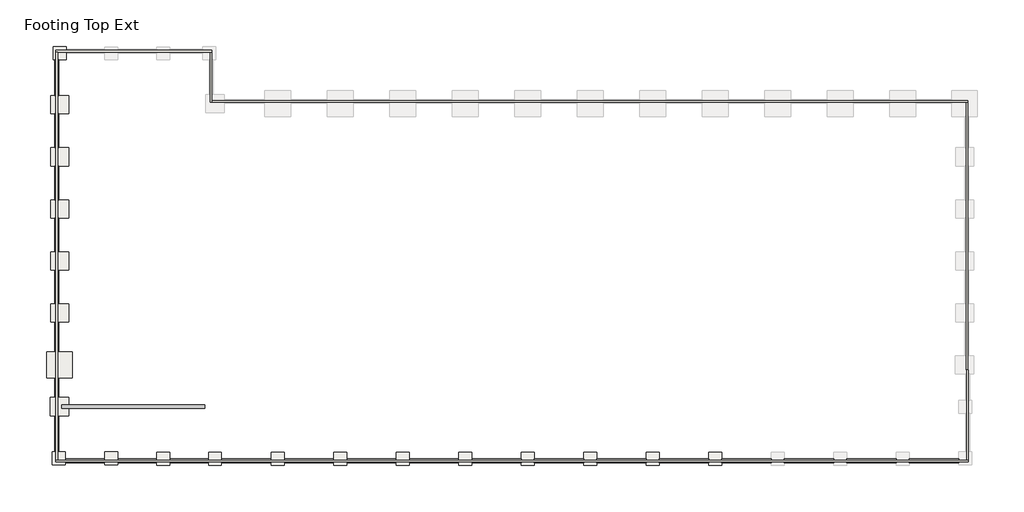
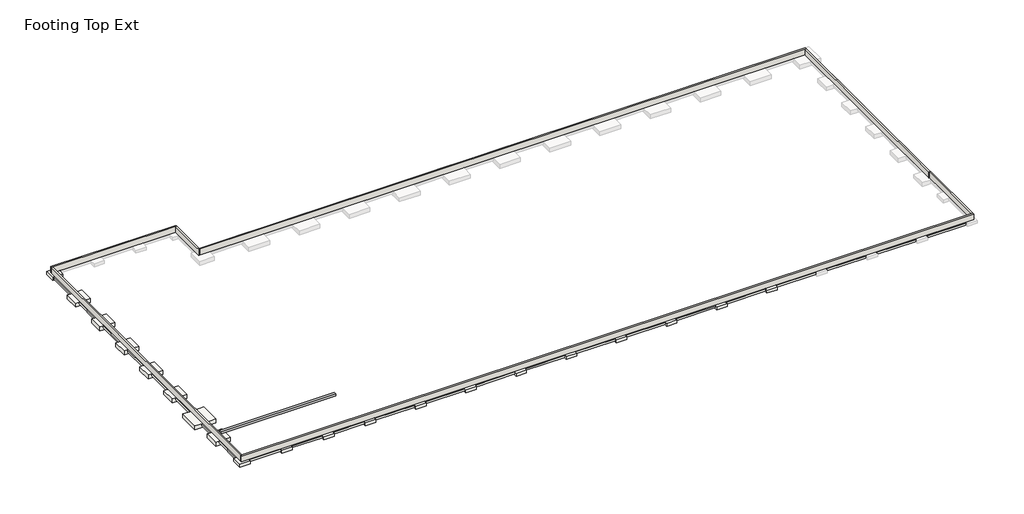
# One storey, part 1 of 2: 20 slabs, 7 walls, 2 footings, 1 beam.
"""IFC4 building model written with IfcOpenShell, lengths in millimetres."""

import ifcopenshell
import ifcopenshell.guid

model = None  # the IFC model being written
_history = None  # IfcOwnerHistory: only IFC2X3 demands one
_inside = {}  # id of a spatial element -> (the spatial element, [elements in it])
_under = {}  # id of a project, library or spatial element -> (it, [spatial elements below it])
_declared = {}  # id of a project -> (the project, [libraries it declares])
_typed = {}  # id of a type object -> (the type object, [elements of that type])
_made_of = {}  # id of a material, layer set ... -> (it, [elements and type objects made of it])


def new_model(schema):
    """Start an empty IFC model of exactly this schema.

    Asked for "IFC4X3", IfcOpenShell would pick the latest addendum, in which some entities
    have other attributes; the version numbers below select the first issue.
    IFC2X3 requires an IfcOwnerHistory on every rooted entity: one is made here for all.
    """
    global model, _history
    if schema == "IFC4X3":
        model = ifcopenshell.file(schema_version=(4, 3, 0, 0))
    else:
        model = ifcopenshell.file(schema=schema)
    _inside.clear()
    _under.clear()
    _declared.clear()
    _typed.clear()
    _made_of.clear()
    _history = None
    if model.schema == "IFC2X3":
        org = make("IfcOrganization", Name="unknown")
        user = make(
            "IfcPersonAndOrganization",
            ThePerson=make("IfcPerson", FamilyName="unknown"),
            TheOrganization=org,
        )
        app = make(
            "IfcApplication",
            ApplicationDeveloper=org,
            Version="unknown",
            ApplicationFullName="unknown",
            ApplicationIdentifier="unknown",
        )
        _history = make(
            "IfcOwnerHistory",
            OwningUser=user,
            OwningApplication=app,
            ChangeAction="ADDED",
            CreationDate=0,
        )
    return model


def make(cls, **values):
    """One entity of the class cls with the attributes given. An attribute that is None is left unset."""
    return model.create_entity(
        cls, **{name: value for name, value in values.items() if value is not None}
    )


def rooted(cls, **values):
    """An entity with a GlobalId (a new one), such as an element, a storey or a relation."""
    return make(cls, GlobalId=ifcopenshell.guid.new(), OwnerHistory=_history, **values)


def si_unit(unit_type, name, prefix=None):
    """IfcSIUnit, for example si_unit("LENGTHUNIT", "METRE", prefix="MILLI")."""
    return make("IfcSIUnit", UnitType=unit_type, Prefix=prefix, Name=name)


def assignment(units):
    """IfcUnitAssignment: the units of a project."""
    return None if units is None else make("IfcUnitAssignment", Units=units)


def point(xyz):
    """IfcCartesianPoint."""
    return None if xyz is None else make("IfcCartesianPoint", Coordinates=xyz)


def direction(xyz):
    """IfcDirection."""
    return None if xyz is None else make("IfcDirection", DirectionRatios=xyz)


def frame(location, z_axis=None, x_axis=None):
    """IfcAxis2Placement3D, a coordinate frame: its origin and axes. An axis left out is left unset."""
    return make(
        "IfcAxis2Placement3D",
        Location=point(location),
        Axis=direction(z_axis),
        RefDirection=direction(x_axis),
    )


def origin():
    """The frame at (0, 0, 0) with its axes left unset."""
    return frame((0.0, 0.0, 0.0))


def place(relative_to, where):
    """IfcLocalPlacement: puts the frame where relative to a parent placement (None: the world)."""
    return make(
        "IfcLocalPlacement", PlacementRelTo=relative_to, RelativePlacement=where
    )


def context(
    kind, dimensions, precision=None, world=None, true_north=None, identifier=None
):
    """IfcGeometricRepresentationContext, for example the 3D "Model" context."""
    return make(
        "IfcGeometricRepresentationContext",
        ContextIdentifier=identifier,
        ContextType=kind,
        CoordinateSpaceDimension=dimensions,
        Precision=precision,
        WorldCoordinateSystem=world,
        TrueNorth=true_north,
    )


def project(units=None, contexts=None):
    """IfcProject with its units and contexts."""
    return rooted(
        "IfcProject",
        Name="project",
        RepresentationContexts=contexts,
        UnitsInContext=assignment(units),
    )


def spatial(cls, under=None, at=None, **own):
    """A site, building, storey or space (cls), placed at a placement, below another one or the project."""
    s = rooted(cls, ObjectPlacement=at, **own)
    if under is not None:
        _under.setdefault(under.id(), (under, []))[1].append(s)
    return s


def polyline(points):
    """IfcPolyline through the points."""
    return make("IfcPolyline", Points=[point(p) for p in points])


def outline(outer, holes=None, kind="AREA"):
    """IfcArbitraryClosedProfileDef: a profile drawn as a closed curve; with holes, ...WithVoids."""
    if holes is None:
        return make("IfcArbitraryClosedProfileDef", ProfileType=kind, OuterCurve=outer)
    return make(
        "IfcArbitraryProfileDefWithVoids",
        ProfileType=kind,
        OuterCurve=outer,
        InnerCurves=holes,
    )


def extrude(swept, where, along, depth):
    """IfcExtrudedAreaSolid: the profile swept, set in the frame where, extruded along a direction by depth."""
    return make(
        "IfcExtrudedAreaSolid",
        SweptArea=swept,
        Position=where,
        ExtrudedDirection=direction(along),
        Depth=depth,
    )


def faces_of(points, faces, orient=None, outer=None):
    """IfcFace entities. A face is a list of loops; a loop is a list of indices into points, from 0.

    orient and outer hold one flag for each loop. By default every Orientation is true, the
    first loop of a face is its IfcFaceOuterBound and the others are IfcFaceBound.
    """
    made = []
    for i, loops in enumerate(faces):
        bounds = []
        for j, loop in enumerate(loops):
            is_outer = j == 0 if outer is None else outer[i][j]
            bounds.append(
                make(
                    "IfcFaceOuterBound" if is_outer else "IfcFaceBound",
                    Bound=make("IfcPolyLoop", Polygon=[points[k] for k in loop]),
                    Orientation=True if orient is None else orient[i][j],
                )
            )
        made.append(make("IfcFace", Bounds=bounds))
    return made


def faceted_brep(points, faces, orient=None, outer=None, voids=None):
    """IfcFacetedBrep: a solid bounded by flat faces; with voids (closed shells), ...WithVoids."""
    shared = [point(p) for p in points]
    hull = make("IfcClosedShell", CfsFaces=faces_of(shared, faces, orient, outer))
    if voids is None:
        return make("IfcFacetedBrep", Outer=hull)
    return make(
        "IfcFacetedBrepWithVoids",
        Outer=hull,
        Voids=[
            make(cls, CfsFaces=faces_of(shared, fs, o, b)) for cls, fs, o, b in voids
        ],
    )


def shape(context_of_items, identifier, shape_type, items):
    """IfcShapeRepresentation: the items that make up one representation, for example the "Body"."""
    return make(
        "IfcShapeRepresentation",
        ContextOfItems=context_of_items,
        RepresentationIdentifier=identifier,
        RepresentationType=shape_type,
        Items=items,
    )


def made_of(thing, what):
    """Note that an element or type object is made of a material, layer set ...; save() writes the relation."""
    if what is not None:
        _made_of.setdefault(what.id(), (what, []))[1].append(thing)
    return thing


def element(
    cls,
    number,
    at=None,
    inside=None,
    cuts=None,
    type_object=None,
    material=None,
    context=None,
    identifier="Body",
    shape_type=None,
    held_by="IfcProductDefinitionShape",
    body=None,
    shapes=None,
    **own,
):
    """One element of the class cls, such as IfcWall. Its Tag is "e" and its number.

    at: its placement. inside: the storey or other place that contains it. cuts: it is an
    opening in that element (IfcRelVoidsElement). A single representation is given by context,
    identifier, shape_type and body (its items); several are given by shapes. held_by: the class
    of the entity that holds the representations. save() writes the other relations.
    """
    e = rooted(cls, Tag="e%d" % number, ObjectPlacement=at, **own)
    if body is not None:
        shapes = [shape(context, identifier, shape_type, body)]
    if shapes is not None:
        e.Representation = make(held_by, Representations=shapes)
    if inside is not None:
        _inside.setdefault(inside.id(), (inside, []))[1].append(e)
    if cuts is not None:
        rooted(
            "IfcRelVoidsElement", RelatingBuildingElement=cuts, RelatedOpeningElement=e
        )
    if type_object is not None:
        _typed.setdefault(type_object.id(), (type_object, []))[1].append(e)
    return made_of(e, material)


def aggregate(whole, parts):
    """IfcRelAggregates: a whole, such as a stair, and the parts it consists of."""
    return rooted("IfcRelAggregates", RelatingObject=whole, RelatedObjects=parts)


def save(model, path):
    """Write the relations noted so far, then the file.

    IfcRelAggregates (storeys below a building ...), IfcRelContainedInSpatialStructure (elements
    in a storey), IfcRelDefinesByType, IfcRelAssociatesMaterial and IfcRelDeclares: one each for
    every whole, place, type object, material and project.
    """
    for whole, parts in _under.values():
        aggregate(whole, parts)
    for where, things in _inside.values():
        rooted(
            "IfcRelContainedInSpatialStructure",
            RelatedElements=things,
            RelatingStructure=where,
        )
    for kind, things in _typed.values():
        rooted("IfcRelDefinesByType", RelatedObjects=things, RelatingType=kind)
    for what, things in _made_of.values():
        rooted("IfcRelAssociatesMaterial", RelatedObjects=things, RelatingMaterial=what)
    for by, libraries in _declared.values():
        rooted("IfcRelDeclares", RelatingContext=by, RelatedDefinitions=libraries)
    model.write(path)


model = new_model("IFC4")

# Units and contexts
model_context = context("Model", 3, world=origin())
ifc_project = project(units=[si_unit("LENGTHUNIT", "METRE", prefix="MILLI")], contexts=[model_context])

# Site, building, storey
site = spatial("IfcSite", under=ifc_project)
building = spatial("IfcBuilding", under=site)
storey = spatial("IfcBuildingStorey", under=building, Name="Footing Top Ext", Elevation=-914.4)

# Beam
placement = place(None, origin())
element("IfcBeam", 1, ObjectType="Concrete-Rectangular Beam : 16 x 12", at=placement, inside=storey, context=model_context, shape_type="SweptSolid", body=[
    extrude(outline(polyline([(321987.9648264, -572404.4391729), (321987.9648264, -572810.8391729), (305208.0898264, -572810.8391729), (305208.0898264, -572404.4391729), (321987.9648264, -572404.4391729)])), frame((0.0, 0.0, -609.6), z_axis=(0.0, 0.0, 1.0), x_axis=(1.0, 0.0, 0.0)), (0.0, 0.0, 1.0), 304.8),
])

# Footings
element("IfcFooting", 2, ObjectType="Bearing Footing - 18\" x 12\"", at=placement, inside=storey, context=model_context, shape_type="SweptSolid", body=[
    extrude(outline(polyline([(305608.1398264, -579216.5913841), (305608.1398264, -578759.3913841), (310230.9398264, -578759.3913841), (310230.9398264, -579216.5913841), (305608.1398264, -579216.5913841)])), frame((0.0, 0.0, -1219.2), z_axis=(0.0, 0.0, 1.0), x_axis=(1.0, 0.0, 0.0)), (0.0, 0.0, 1.0), 304.8),
    extrude(outline(polyline([(311754.9398264, -579216.5913841), (311754.9398264, -578759.3913841), (316361.8648264, -578759.3913841), (316361.8648264, -579216.5913841), (311754.9398264, -579216.5913841)])), frame((0.0, 0.0, -1219.2), z_axis=(0.0, 0.0, 1.0), x_axis=(1.0, 0.0, 0.0)), (0.0, 0.0, 1.0), 304.8),
    extrude(outline(polyline([(317885.8648264, -579216.5913841), (317885.8648264, -578759.3913841), (322457.8648264, -578759.3913841), (322457.8648264, -579216.5913841), (317885.8648264, -579216.5913841)])), frame((0.0, 0.0, -1219.2), z_axis=(0.0, 0.0, 1.0), x_axis=(1.0, 0.0, 0.0)), (0.0, 0.0, 1.0), 304.8),
    extrude(outline(polyline([(323981.8648264, -579216.5913841), (323981.8648264, -578759.3913841), (329839.7398264, -578759.3913841), (329839.7398264, -579216.5913841), (323981.8648264, -579216.5913841)])), frame((0.0, 0.0, -1219.2), z_axis=(0.0, 0.0, 1.0), x_axis=(1.0, 0.0, 0.0)), (0.0, 0.0, 1.0), 304.8),
    extrude(outline(polyline([(331363.7398264, -579216.5913841), (331363.7398264, -578759.3913841), (337193.0398264, -578759.3913841), (337193.0398264, -579216.5913841), (331363.7398264, -579216.5913841)])), frame((0.0, 0.0, -1219.2), z_axis=(0.0, 0.0, 1.0), x_axis=(1.0, 0.0, 0.0)), (0.0, 0.0, 1.0), 304.8),
    extrude(outline(polyline([(338717.0398264, -579216.5913841), (338717.0398264, -578759.3913841), (344546.3398264, -578759.3913841), (344546.3398264, -579216.5913841), (338717.0398264, -579216.5913841)])), frame((0.0, 0.0, -1219.2), z_axis=(0.0, 0.0, 1.0), x_axis=(1.0, 0.0, 0.0)), (0.0, 0.0, 1.0), 304.8),
    extrude(outline(polyline([(346070.3398264, -579216.5913841), (346070.3398264, -578759.3913841), (351899.6398264, -578759.3913841), (351899.6398264, -579216.5913841), (346070.3398264, -579216.5913841)])), frame((0.0, 0.0, -1219.2), z_axis=(0.0, 0.0, 1.0), x_axis=(1.0, 0.0, 0.0)), (0.0, 0.0, 1.0), 304.8),
    extrude(outline(polyline([(353423.6398264, -579216.5913841), (353423.6398264, -578759.3913841), (359252.9398264, -578759.3913841), (359252.9398264, -579216.5913841), (353423.6398264, -579216.5913841)])), frame((0.0, 0.0, -1219.2), z_axis=(0.0, 0.0, 1.0), x_axis=(1.0, 0.0, 0.0)), (0.0, 0.0, 1.0), 304.8),
    extrude(outline(polyline([(360776.9398264, -579216.5913841), (360776.9398264, -578759.3913841), (366606.2398264, -578759.3913841), (366606.2398264, -579216.5913841), (360776.9398264, -579216.5913841)])), frame((0.0, 0.0, -1219.2), z_axis=(0.0, 0.0, 1.0), x_axis=(1.0, 0.0, 0.0)), (0.0, 0.0, 1.0), 304.8),
    extrude(outline(polyline([(368130.2398264, -579216.5913841), (368130.2398264, -578759.3913841), (373959.5398264, -578759.3913841), (373959.5398264, -579216.5913841), (368130.2398264, -579216.5913841)])), frame((0.0, 0.0, -1219.2), z_axis=(0.0, 0.0, 1.0), x_axis=(1.0, 0.0, 0.0)), (0.0, 0.0, 1.0), 304.8),
    extrude(outline(polyline([(375483.5398264, -579216.5913841), (375483.5398264, -578759.3913841), (381312.8398264, -578759.3913841), (381312.8398264, -579216.5913841), (375483.5398264, -579216.5913841)])), frame((0.0, 0.0, -1219.2), z_axis=(0.0, 0.0, 1.0), x_axis=(1.0, 0.0, 0.0)), (0.0, 0.0, 1.0), 304.8),
    extrude(outline(polyline([(382836.8398264, -579216.5913841), (382836.8398264, -578759.3913841), (388666.1398264, -578759.3913841), (388666.1398264, -579216.5913841), (382836.8398264, -579216.5913841)])), frame((0.0, 0.0, -1219.2), z_axis=(0.0, 0.0, 1.0), x_axis=(1.0, 0.0, 0.0)), (0.0, 0.0, 1.0), 304.8),
    extrude(outline(polyline([(390190.1398264, -579216.5913841), (390190.1398264, -578759.3913841), (396019.4398264, -578759.3913841), (396019.4398264, -579216.5913841), (390190.1398264, -579216.5913841)])), frame((0.0, 0.0, -1219.2), z_axis=(0.0, 0.0, 1.0), x_axis=(1.0, 0.0, 0.0)), (0.0, 0.0, 1.0), 304.8),
    extrude(outline(polyline([(397543.4398264, -579216.5913841), (397543.4398264, -578759.3913841), (403372.7398264, -578759.3913841), (403372.7398264, -579216.5913841), (397543.4398264, -579216.5913841)])), frame((0.0, 0.0, -1219.2), z_axis=(0.0, 0.0, 1.0), x_axis=(1.0, 0.0, 0.0)), (0.0, 0.0, 1.0), 304.8),
    extrude(outline(polyline([(404896.7398264, -579216.5913841), (404896.7398264, -578759.3913841), (410700.6398264, -578759.3913841), (410700.6398264, -579216.5913841), (404896.7398264, -579216.5913841)])), frame((0.0, 0.0, -1219.2), z_axis=(0.0, 0.0, 1.0), x_axis=(1.0, 0.0, 0.0)), (0.0, 0.0, 1.0), 304.8),
])
element("IfcFooting", 3, ObjectType="Bearing Footing - 18\" x 12\"", at=placement, inside=storey, context=model_context, shape_type="SweptSolid", body=[
    extrude(outline(polyline([(304369.8898264, -531712.2413841), (304827.0898264, -531712.2413841), (304827.0898264, -535985.7913841), (304369.8898264, -535985.7913841), (304369.8898264, -531712.2413841)])), frame((0.0, 0.0, -1219.2), z_axis=(0.0, 0.0, 1.0), x_axis=(1.0, 0.0, 0.0)), (0.0, 0.0, 1.0), 304.8),
    extrude(outline(polyline([(304369.8898264, -538119.3913841), (304827.0898264, -538119.3913841), (304827.0898264, -542113.5413841), (304369.8898264, -542113.5413841), (304369.8898264, -538119.3913841)])), frame((0.0, 0.0, -1219.2), z_axis=(0.0, 0.0, 1.0), x_axis=(1.0, 0.0, 0.0)), (0.0, 0.0, 1.0), 304.8),
    extrude(outline(polyline([(304369.8898264, -544247.1413841), (304827.0898264, -544247.1413841), (304827.0898264, -548241.2913841), (304369.8898264, -548241.2913841), (304369.8898264, -544247.1413841)])), frame((0.0, 0.0, -1219.2), z_axis=(0.0, 0.0, 1.0), x_axis=(1.0, 0.0, 0.0)), (0.0, 0.0, 1.0), 304.8),
    extrude(outline(polyline([(304369.8898264, -550374.8913841), (304827.0898264, -550374.8913841), (304827.0898264, -554369.0413841), (304369.8898264, -554369.0413841), (304369.8898264, -550374.8913841)])), frame((0.0, 0.0, -1219.2), z_axis=(0.0, 0.0, 1.0), x_axis=(1.0, 0.0, 0.0)), (0.0, 0.0, 1.0), 304.8),
    extrude(outline(polyline([(304369.8898264, -556502.6413841), (304827.0898264, -556502.6413841), (304827.0898264, -560496.7913841), (304369.8898264, -560496.7913841), (304369.8898264, -556502.6413841)])), frame((0.0, 0.0, -1219.2), z_axis=(0.0, 0.0, 1.0), x_axis=(1.0, 0.0, 0.0)), (0.0, 0.0, 1.0), 304.8),
    extrude(outline(polyline([(304369.8898264, -562630.3913841), (304827.0898264, -562630.3913841), (304827.0898264, -566167.3413841), (304369.8898264, -566167.3413841), (304369.8898264, -562630.3913841)])), frame((0.0, 0.0, -1219.2), z_axis=(0.0, 0.0, 1.0), x_axis=(1.0, 0.0, 0.0)), (0.0, 0.0, 1.0), 304.8),
    extrude(outline(polyline([(304369.8898264, -569215.3413841), (304827.0898264, -569215.3413841), (304827.0898264, -571526.7413841), (304369.8898264, -571526.7413841), (304369.8898264, -569215.3413841)])), frame((0.0, 0.0, -1219.2), z_axis=(0.0, 0.0, 1.0), x_axis=(1.0, 0.0, 0.0)), (0.0, 0.0, 1.0), 304.8),
    extrude(outline(polyline([(304369.8898264, -573660.3413841), (304827.0898264, -573660.3413841), (304827.0898264, -577933.8913841), (304369.8898264, -577933.8913841), (304369.8898264, -573660.3413841)])), frame((0.0, 0.0, -1219.2), z_axis=(0.0, 0.0, 1.0), x_axis=(1.0, 0.0, 0.0)), (0.0, 0.0, 1.0), 304.8),
])

# Slabs
element("IfcSlab", 4, ObjectType="Footing-Rectangular : F10", at=placement, inside=storey, context=model_context, shape_type="Brep", body=[
    faceted_brep([(306452.6898264, -566167.3413841, -914.4), (304827.0898264, -566167.3413841, -914.4), (304369.8898264, -566167.3413841, -914.4), (303404.6898264, -566167.3413841, -914.4), (303404.6898264, -569215.3413841, -914.4), (304369.8898264, -569215.3413841, -914.4), (304827.0898264, -569215.3413841, -914.4), (306452.6898264, -569215.3413841, -914.4), (306452.6898264, -566167.3413841, -1524.0), (306452.6898264, -569215.3413841, -1524.0), (303404.6898264, -569215.3413841, -1524.0), (303404.6898264, -566167.3413841, -1524.0)], [[[0, 1, 2, 3, 4, 5, 6, 7]], [[8, 9, 10, 11]], [[3, 2, 1, 0, 8, 11]], [[4, 3, 11, 10]], [[7, 6, 5, 4, 10, 9]], [[0, 7, 9, 8]]]),
])
element("IfcSlab", 5, ObjectType="Footing-Rectangular : F5", at=placement, inside=storey, context=model_context, shape_type="Brep", body=[
    faceted_brep([(305697.0398264, -530188.2413841, -914.4), (304173.0398264, -530188.2413841, -914.4), (304173.0398264, -531712.2413841, -914.4), (304369.8898264, -531712.2413841, -914.4), (304827.0898264, -531712.2413841, -914.4), (305697.0398264, -531712.2413841, -914.4), (305697.0398264, -530975.6413841, -914.4), (305697.0398264, -530518.4413841, -914.4), (305697.0398264, -530188.2413841, -1371.6), (305697.0398264, -531712.2413841, -1371.6), (304173.0398264, -531712.2413841, -1371.6), (304173.0398264, -530188.2413841, -1371.6)], [[[0, 1, 2, 3, 4, 5, 6, 7]], [[8, 9, 10, 11]], [[1, 0, 8, 11]], [[2, 1, 11, 10]], [[5, 4, 3, 2, 10, 9]], [[0, 7, 6, 5, 9, 8]]]),
])
element("IfcSlab", 6, ObjectType="Footing-Rectangular : F5", at=placement, inside=storey, context=model_context, shape_type="Brep", body=[
    faceted_brep([(305608.1398264, -577933.8913841, -914.4), (304827.0898264, -577933.8913841, -914.4), (304369.8898264, -577933.8913841, -914.4), (304084.1398264, -577933.8913841, -914.4), (304084.1398264, -579457.8913841, -914.4), (305608.1398264, -579457.8913841, -914.4), (305608.1398264, -579216.5913841, -914.4), (305608.1398264, -578759.3913841, -914.4), (305608.1398264, -577933.8913841, -1371.6), (305608.1398264, -579457.8913841, -1371.6), (304084.1398264, -579457.8913841, -1371.6), (304084.1398264, -577933.8913841, -1371.6)], [[[0, 1, 2, 3, 4, 5, 6, 7]], [[8, 9, 10, 11]], [[3, 2, 1, 0, 8, 11]], [[4, 3, 11, 10]], [[5, 4, 10, 9]], [[0, 7, 6, 5, 9, 8]]]),
])
element("IfcSlab", 7, ObjectType="Footing-Rectangular : F5", at=placement, inside=storey, context=model_context, shape_type="Brep", body=[
    faceted_brep([(311754.9398264, -577927.5413841, -914.4), (310230.9398264, -577927.5413841, -914.4), (310230.9398264, -578759.3913841, -914.4), (310230.9398264, -579216.5913841, -914.4), (310230.9398264, -579451.5413841, -914.4), (311754.9398264, -579451.5413841, -914.4), (311754.9398264, -579216.5913841, -914.4), (311754.9398264, -578759.3913841, -914.4), (311754.9398264, -577927.5413841, -1371.6), (311754.9398264, -579451.5413841, -1371.6), (310230.9398264, -579451.5413841, -1371.6), (310230.9398264, -577927.5413841, -1371.6)], [[[0, 1, 2, 3, 4, 5, 6, 7]], [[8, 9, 10, 11]], [[1, 0, 8, 11]], [[4, 3, 2, 1, 11, 10]], [[5, 4, 10, 9]], [[0, 7, 6, 5, 9, 8]]]),
])
element("IfcSlab", 8, ObjectType="Footing-Rectangular : F5", at=placement, inside=storey, context=model_context, shape_type="Brep", body=[
    faceted_brep([(317885.8648264, -577971.9913841, -914.4), (316361.8648264, -577971.9913841, -914.4), (316361.8648264, -578759.3913841, -914.4), (316361.8648264, -579216.5913841, -914.4), (316361.8648264, -579495.9913841, -914.4), (317885.8648264, -579495.9913841, -914.4), (317885.8648264, -579216.5913841, -914.4), (317885.8648264, -578759.3913841, -914.4), (317885.8648264, -577971.9913841, -1371.6), (317885.8648264, -579495.9913841, -1371.6), (316361.8648264, -579495.9913841, -1371.6), (316361.8648264, -577971.9913841, -1371.6)], [[[0, 1, 2, 3, 4, 5, 6, 7]], [[8, 9, 10, 11]], [[1, 0, 8, 11]], [[4, 3, 2, 1, 11, 10]], [[5, 4, 10, 9]], [[0, 7, 6, 5, 9, 8]]]),
])
element("IfcSlab", 9, ObjectType="Footing-Rectangular : F5", at=placement, inside=storey, context=model_context, shape_type="Brep", body=[
    faceted_brep([(323981.8648264, -577971.9913841, -914.4), (322457.8648264, -577971.9913841, -914.4), (322457.8648264, -578759.3913841, -914.4), (322457.8648264, -579216.5913841, -914.4), (322457.8648264, -579495.9913841, -914.4), (323981.8648264, -579495.9913841, -914.4), (323981.8648264, -579216.5913841, -914.4), (323981.8648264, -578759.3913841, -914.4), (323981.8648264, -577971.9913841, -1371.6), (323981.8648264, -579495.9913841, -1371.6), (322457.8648264, -579495.9913841, -1371.6), (322457.8648264, -577971.9913841, -1371.6)], [[[0, 1, 2, 3, 4, 5, 6, 7]], [[8, 9, 10, 11]], [[1, 0, 8, 11]], [[4, 3, 2, 1, 11, 10]], [[5, 4, 10, 9]], [[0, 7, 6, 5, 9, 8]]]),
])
element("IfcSlab", 10, ObjectType="Footing-Rectangular : F5", at=placement, inside=storey, context=model_context, shape_type="Brep", body=[
    faceted_brep([(331363.7398264, -577978.3413841, -914.4), (329839.7398264, -577978.3413841, -914.4), (329839.7398264, -578759.3913841, -914.4), (329839.7398264, -579216.5913841, -914.4), (329839.7398264, -579502.3413841, -914.4), (331363.7398264, -579502.3413841, -914.4), (331363.7398264, -579216.5913841, -914.4), (331363.7398264, -578759.3913841, -914.4), (331363.7398264, -577978.3413841, -1371.6), (331363.7398264, -579502.3413841, -1371.6), (329839.7398264, -579502.3413841, -1371.6), (329839.7398264, -577978.3413841, -1371.6)], [[[0, 1, 2, 3, 4, 5, 6, 7]], [[8, 9, 10, 11]], [[1, 0, 8, 11]], [[4, 3, 2, 1, 11, 10]], [[5, 4, 10, 9]], [[0, 7, 6, 5, 9, 8]]]),
])
element("IfcSlab", 11, ObjectType="Footing-Rectangular : F5", at=placement, inside=storey, context=model_context, shape_type="Brep", body=[
    faceted_brep([(338717.0398264, -577978.3413841, -914.4), (337193.0398264, -577978.3413841, -914.4), (337193.0398264, -578759.3913841, -914.4), (337193.0398264, -579216.5913841, -914.4), (337193.0398264, -579502.3413841, -914.4), (338717.0398264, -579502.3413841, -914.4), (338717.0398264, -579216.5913841, -914.4), (338717.0398264, -578759.3913841, -914.4), (338717.0398264, -577978.3413841, -1371.6), (338717.0398264, -579502.3413841, -1371.6), (337193.0398264, -579502.3413841, -1371.6), (337193.0398264, -577978.3413841, -1371.6)], [[[0, 1, 2, 3, 4, 5, 6, 7]], [[8, 9, 10, 11]], [[1, 0, 8, 11]], [[4, 3, 2, 1, 11, 10]], [[5, 4, 10, 9]], [[0, 7, 6, 5, 9, 8]]]),
])
element("IfcSlab", 12, ObjectType="Footing-Rectangular : F5", at=placement, inside=storey, context=model_context, shape_type="Brep", body=[
    faceted_brep([(346070.3398264, -577978.3413841, -914.4), (344546.3398264, -577978.3413841, -914.4), (344546.3398264, -578759.3913841, -914.4), (344546.3398264, -579216.5913841, -914.4), (344546.3398264, -579502.3413841, -914.4), (346070.3398264, -579502.3413841, -914.4), (346070.3398264, -579216.5913841, -914.4), (346070.3398264, -578759.3913841, -914.4), (346070.3398264, -577978.3413841, -1371.6), (346070.3398264, -579502.3413841, -1371.6), (344546.3398264, -579502.3413841, -1371.6), (344546.3398264, -577978.3413841, -1371.6)], [[[0, 1, 2, 3, 4, 5, 6, 7]], [[8, 9, 10, 11]], [[1, 0, 8, 11]], [[4, 3, 2, 1, 11, 10]], [[5, 4, 10, 9]], [[0, 7, 6, 5, 9, 8]]]),
])
element("IfcSlab", 13, ObjectType="Footing-Rectangular : F5", at=placement, inside=storey, context=model_context, shape_type="Brep", body=[
    faceted_brep([(353423.6398264, -577978.3413841, -914.4), (351899.6398264, -577978.3413841, -914.4), (351899.6398264, -578759.3913841, -914.4), (351899.6398264, -579216.5913841, -914.4), (351899.6398264, -579502.3413841, -914.4), (353423.6398264, -579502.3413841, -914.4), (353423.6398264, -579216.5913841, -914.4), (353423.6398264, -578759.3913841, -914.4), (353423.6398264, -577978.3413841, -1371.6), (353423.6398264, -579502.3413841, -1371.6), (351899.6398264, -579502.3413841, -1371.6), (351899.6398264, -577978.3413841, -1371.6)], [[[0, 1, 2, 3, 4, 5, 6, 7]], [[8, 9, 10, 11]], [[1, 0, 8, 11]], [[4, 3, 2, 1, 11, 10]], [[5, 4, 10, 9]], [[0, 7, 6, 5, 9, 8]]]),
])
element("IfcSlab", 14, ObjectType="Footing-Rectangular : F5", at=placement, inside=storey, context=model_context, shape_type="Brep", body=[
    faceted_brep([(360776.9398264, -577978.3413841, -914.4), (359252.9398264, -577978.3413841, -914.4), (359252.9398264, -578759.3913841, -914.4), (359252.9398264, -579216.5913841, -914.4), (359252.9398264, -579502.3413841, -914.4), (360776.9398264, -579502.3413841, -914.4), (360776.9398264, -579216.5913841, -914.4), (360776.9398264, -578759.3913841, -914.4), (360776.9398264, -577978.3413841, -1371.6), (360776.9398264, -579502.3413841, -1371.6), (359252.9398264, -579502.3413841, -1371.6), (359252.9398264, -577978.3413841, -1371.6)], [[[0, 1, 2, 3, 4, 5, 6, 7]], [[8, 9, 10, 11]], [[1, 0, 8, 11]], [[4, 3, 2, 1, 11, 10]], [[5, 4, 10, 9]], [[0, 7, 6, 5, 9, 8]]]),
])
element("IfcSlab", 15, ObjectType="Footing-Rectangular : F5", at=placement, inside=storey, context=model_context, shape_type="Brep", body=[
    faceted_brep([(368130.2398264, -577978.3413841, -914.4), (366606.2398264, -577978.3413841, -914.4), (366606.2398264, -578759.3913841, -914.4), (366606.2398264, -579216.5913841, -914.4), (366606.2398264, -579502.3413841, -914.4), (368130.2398264, -579502.3413841, -914.4), (368130.2398264, -579216.5913841, -914.4), (368130.2398264, -578759.3913841, -914.4), (368130.2398264, -577978.3413841, -1371.6), (368130.2398264, -579502.3413841, -1371.6), (366606.2398264, -579502.3413841, -1371.6), (366606.2398264, -577978.3413841, -1371.6)], [[[0, 1, 2, 3, 4, 5, 6, 7]], [[8, 9, 10, 11]], [[1, 0, 8, 11]], [[4, 3, 2, 1, 11, 10]], [[5, 4, 10, 9]], [[0, 7, 6, 5, 9, 8]]]),
])
element("IfcSlab", 16, ObjectType="Footing-Rectangular : F5", at=placement, inside=storey, context=model_context, shape_type="Brep", body=[
    faceted_brep([(375483.5398264, -577978.3413841, -914.4), (373959.5398264, -577978.3413841, -914.4), (373959.5398264, -578759.3913841, -914.4), (373959.5398264, -579216.5913841, -914.4), (373959.5398264, -579502.3413841, -914.4), (375483.5398264, -579502.3413841, -914.4), (375483.5398264, -579216.5913841, -914.4), (375483.5398264, -578759.3913841, -914.4), (375483.5398264, -577978.3413841, -1371.6), (375483.5398264, -579502.3413841, -1371.6), (373959.5398264, -579502.3413841, -1371.6), (373959.5398264, -577978.3413841, -1371.6)], [[[0, 1, 2, 3, 4, 5, 6, 7]], [[8, 9, 10, 11]], [[1, 0, 8, 11]], [[4, 3, 2, 1, 11, 10]], [[5, 4, 10, 9]], [[0, 7, 6, 5, 9, 8]]]),
])
element("IfcSlab", 17, ObjectType="Footing-Rectangular : F5", at=placement, inside=storey, context=model_context, shape_type="Brep", body=[
    faceted_brep([(382836.8398264, -577978.3413841, -914.4), (381312.8398264, -577978.3413841, -914.4), (381312.8398264, -578759.3913841, -914.4), (381312.8398264, -579216.5913841, -914.4), (381312.8398264, -579502.3413841, -914.4), (382836.8398264, -579502.3413841, -914.4), (382836.8398264, -579216.5913841, -914.4), (382836.8398264, -578759.3913841, -914.4), (382836.8398264, -577978.3413841, -1371.6), (382836.8398264, -579502.3413841, -1371.6), (381312.8398264, -579502.3413841, -1371.6), (381312.8398264, -577978.3413841, -1371.6)], [[[0, 1, 2, 3, 4, 5, 6, 7]], [[8, 9, 10, 11]], [[1, 0, 8, 11]], [[4, 3, 2, 1, 11, 10]], [[5, 4, 10, 9]], [[0, 7, 6, 5, 9, 8]]]),
])
element("IfcSlab", 18, ObjectType="Footing-Rectangular : F7", at=placement, inside=storey, context=model_context, shape_type="Brep", body=[
    faceted_brep([(306020.8898264, -535985.7913841, -914.4), (304827.0898264, -535985.7913841, -914.4), (304369.8898264, -535985.7913841, -914.4), (303887.2898264, -535985.7913841, -914.4), (303887.2898264, -538119.3913841, -914.4), (304369.8898264, -538119.3913841, -914.4), (304827.0898264, -538119.3913841, -914.4), (306020.8898264, -538119.3913841, -914.4), (306020.8898264, -535985.7913841, -1524.0), (306020.8898264, -538119.3913841, -1524.0), (303887.2898264, -538119.3913841, -1524.0), (303887.2898264, -535985.7913841, -1524.0)], [[[0, 1, 2, 3, 4, 5, 6, 7]], [[8, 9, 10, 11]], [[3, 2, 1, 0, 8, 11]], [[4, 3, 11, 10]], [[7, 6, 5, 4, 10, 9]], [[0, 7, 9, 8]]]),
])
element("IfcSlab", 19, ObjectType="Footing-Rectangular : F7", at=placement, inside=storey, context=model_context, shape_type="Brep", body=[
    faceted_brep([(306020.8898264, -542113.5413841, -914.4), (304827.0898264, -542113.5413841, -914.4), (304369.8898264, -542113.5413841, -914.4), (303887.2898264, -542113.5413841, -914.4), (303887.2898264, -544247.1413841, -914.4), (304369.8898264, -544247.1413841, -914.4), (304827.0898264, -544247.1413841, -914.4), (306020.8898264, -544247.1413841, -914.4), (306020.8898264, -542113.5413841, -1524.0), (306020.8898264, -544247.1413841, -1524.0), (303887.2898264, -544247.1413841, -1524.0), (303887.2898264, -542113.5413841, -1524.0)], [[[0, 1, 2, 3, 4, 5, 6, 7]], [[8, 9, 10, 11]], [[3, 2, 1, 0, 8, 11]], [[4, 3, 11, 10]], [[7, 6, 5, 4, 10, 9]], [[0, 7, 9, 8]]]),
])
element("IfcSlab", 20, ObjectType="Footing-Rectangular : F7", at=placement, inside=storey, context=model_context, shape_type="Brep", body=[
    faceted_brep([(306020.8898264, -548241.2913841, -914.4), (304827.0898264, -548241.2913841, -914.4), (304369.8898264, -548241.2913841, -914.4), (303887.2898264, -548241.2913841, -914.4), (303887.2898264, -550374.8913841, -914.4), (304369.8898264, -550374.8913841, -914.4), (304827.0898264, -550374.8913841, -914.4), (306020.8898264, -550374.8913841, -914.4), (306020.8898264, -548241.2913841, -1524.0), (306020.8898264, -550374.8913841, -1524.0), (303887.2898264, -550374.8913841, -1524.0), (303887.2898264, -548241.2913841, -1524.0)], [[[0, 1, 2, 3, 4, 5, 6, 7]], [[8, 9, 10, 11]], [[3, 2, 1, 0, 8, 11]], [[4, 3, 11, 10]], [[7, 6, 5, 4, 10, 9]], [[0, 7, 9, 8]]]),
])
element("IfcSlab", 21, ObjectType="Footing-Rectangular : F7", at=placement, inside=storey, context=model_context, shape_type="Brep", body=[
    faceted_brep([(306020.8898264, -554369.0413841, -914.4), (304827.0898264, -554369.0413841, -914.4), (304369.8898264, -554369.0413841, -914.4), (303887.2898264, -554369.0413841, -914.4), (303887.2898264, -556502.6413841, -914.4), (304369.8898264, -556502.6413841, -914.4), (304827.0898264, -556502.6413841, -914.4), (306020.8898264, -556502.6413841, -914.4), (306020.8898264, -554369.0413841, -1524.0), (306020.8898264, -556502.6413841, -1524.0), (303887.2898264, -556502.6413841, -1524.0), (303887.2898264, -554369.0413841, -1524.0)], [[[0, 1, 2, 3, 4, 5, 6, 7]], [[8, 9, 10, 11]], [[3, 2, 1, 0, 8, 11]], [[4, 3, 11, 10]], [[7, 6, 5, 4, 10, 9]], [[0, 7, 9, 8]]]),
])
element("IfcSlab", 22, ObjectType="Footing-Rectangular : F7", at=placement, inside=storey, context=model_context, shape_type="Brep", body=[
    faceted_brep([(306020.8898264, -560496.7913841, -914.4), (304827.0898264, -560496.7913841, -914.4), (304369.8898264, -560496.7913841, -914.4), (303887.2898264, -560496.7913841, -914.4), (303887.2898264, -562630.3913841, -914.4), (304369.8898264, -562630.3913841, -914.4), (304827.0898264, -562630.3913841, -914.4), (306020.8898264, -562630.3913841, -914.4), (306020.8898264, -560496.7913841, -1524.0), (306020.8898264, -562630.3913841, -1524.0), (303887.2898264, -562630.3913841, -1524.0), (303887.2898264, -560496.7913841, -1524.0)], [[[0, 1, 2, 3, 4, 5, 6, 7]], [[8, 9, 10, 11]], [[3, 2, 1, 0, 8, 11]], [[4, 3, 11, 10]], [[7, 6, 5, 4, 10, 9]], [[0, 7, 9, 8]]]),
])
element("IfcSlab", 23, ObjectType="Footing-Rectangular : F7", at=placement, inside=storey, context=model_context, shape_type="Brep", body=[
    faceted_brep([(305995.4898264, -571526.7413841, -914.4), (304827.0898264, -571526.7413841, -914.4), (304369.8898264, -571526.7413841, -914.4), (303861.8898264, -571526.7413841, -914.4), (303861.8898264, -573660.3413841, -914.4), (304369.8898264, -573660.3413841, -914.4), (304827.0898264, -573660.3413841, -914.4), (305995.4898264, -573660.3413841, -914.4), (305995.4898264, -571526.7413841, -1524.0), (305995.4898264, -573660.3413841, -1524.0), (303861.8898264, -573660.3413841, -1524.0), (303861.8898264, -571526.7413841, -1524.0)], [[[0, 1, 2, 3, 4, 5, 6, 7]], [[8, 9, 10, 11]], [[3, 2, 1, 0, 8, 11]], [[4, 3, 11, 10]], [[7, 6, 5, 4, 10, 9]], [[0, 7, 9, 8]]]),
])

# Walls
element("IfcWall", 24, ObjectType="Frost Wall - 8\" Concrete", at=placement, inside=storey, context=model_context, shape_type="Brep", body=[
    faceted_brep([(304496.8898264, -530848.6413841, -914.4), (304681.0398264, -530848.6413841, -914.4), (322664.2398264, -530848.6413841, -914.4), (322867.4398264, -530848.6413841, -914.4), (322867.4398264, -530848.6413841, -152.4), (322867.4398264, -530848.6413841, 0.0), (304496.8898264, -530848.6413841, 0.0), (304496.8898264, -530848.6413841, -152.4), (304496.8898264, -530645.4413841, -914.4), (304496.8898264, -530645.4413841, 0.0), (322867.4398264, -530645.4413841, 0.0), (322867.4398264, -530645.4413841, -914.4)], [[[0, 1, 2, 3, 4, 5, 6, 7]], [[8, 9, 10, 11]], [[3, 2, 1, 0, 8, 11]], [[6, 5, 10, 9]], [[5, 4, 3, 11, 10]], [[0, 7, 6, 9, 8]]]),
])
element("IfcWall", 25, ObjectType="Frost Wall - 8\" Concrete", at=placement, inside=storey, context=model_context, shape_type="Brep", body=[
    faceted_brep([(322664.2398264, -530848.6413841, -914.4), (322664.2398264, -536760.4913841, -914.4), (322664.2398264, -536760.4913841, -152.4), (322664.2398264, -536760.4913841, 0.0), (322664.2398264, -536106.6816264, 0.0), (322664.2398264, -530848.6413841, 0.0), (322664.2398264, -530848.6413841, -152.4), (322867.4398264, -536760.4913841, -914.4), (322867.4398264, -536557.2913841, -914.4), (322867.4398264, -530848.6413841, -914.4), (322867.4398264, -530848.6413841, 0.0), (322867.4398264, -536557.2913841, 0.0), (322867.4398264, -536760.4913841, 0.0), (322867.4398264, -536760.4913841, -152.4)], [[[0, 1, 2, 3, 4, 5, 6]], [[7, 8, 9, 10, 11, 12, 13]], [[1, 0, 9, 8, 7]], [[12, 11, 10, 5, 4, 3]], [[5, 10, 9, 0, 6]], [[1, 7, 13, 12, 3, 2]]]),
])
element("IfcWall", 26, ObjectType="Frost Wall - 8\" Concrete", at=placement, inside=storey, context=model_context, shape_type="Brep", body=[
    faceted_brep([(322867.4398264, -536760.4913841, -914.4), (411564.2398264, -536760.4913841, -914.4), (411767.4398264, -536760.4913841, -914.4), (411767.4398264, -536760.4913841, 0.0), (411564.2398264, -536760.4913841, 0.0), (322867.4398264, -536760.4913841, 0.0), (322867.4398264, -536760.4913841, -152.4), (411767.4398264, -536557.2913841, -914.4), (322867.4398264, -536557.2913841, -914.4), (322867.4398264, -536557.2913841, 0.0), (411767.4398264, -536557.2913841, 0.0)], [[[0, 1, 2, 3, 4, 5, 6]], [[7, 8, 9, 10]], [[2, 1, 0, 8, 7]], [[10, 9, 5, 4, 3]], [[5, 9, 8, 0, 6]], [[3, 2, 7, 10]]]),
])
element("IfcWall", 27, ObjectType="Frost Wall - 8\" Concrete", at=placement, inside=storey, context=model_context, shape_type="SweptSolid", body=[
    extrude(outline(polyline([(411564.2398264, -568288.2413841), (411564.2398264, -536760.4913841), (411767.4398264, -536760.4913841), (411767.4398264, -568288.2413841), (411564.2398264, -568288.2413841)])), frame((0.0, 0.0, -914.4), z_axis=(0.0, 0.0, 1.0), x_axis=(1.0, 0.0, 0.0)), (0.0, 0.0, 1.0), 914.4),
])
element("IfcWall", 28, ObjectType="Frost Wall - 8\" Concrete", at=placement, inside=storey, context=model_context, shape_type="Brep", body=[
    faceted_brep([(411856.3398264, -578886.3913841, -914.4), (411653.1398264, -578886.3913841, -914.4), (304700.0898264, -578886.3913841, -914.4), (304496.8898264, -578886.3913841, -914.4), (304496.8898264, -578886.3913841, 0.0), (304700.0898264, -578886.3913841, 0.0), (411653.1398264, -578886.3913841, 0.0), (411856.3398264, -578886.3913841, 0.0), (411856.3398264, -579089.5913841, -914.4), (411856.3398264, -579089.5913841, 0.0), (304496.8898264, -579089.5913841, 0.0), (304496.8898264, -579089.5913841, -914.4)], [[[0, 1, 2, 3, 4, 5, 6, 7]], [[8, 9, 10, 11]], [[3, 2, 1, 0, 8, 11]], [[7, 6, 5, 4, 10, 9]], [[4, 3, 11, 10]], [[0, 7, 9, 8]]]),
])
element("IfcWall", 29, ObjectType="Frost Wall - 8\" Concrete", at=placement, inside=storey, context=model_context, shape_type="SweptSolid", body=[
    extrude(outline(polyline([(304700.0898264, -530848.6413841), (304700.0898264, -578886.3913841), (304496.8898264, -578886.3913841), (304496.8898264, -530848.6413841), (304700.0898264, -530848.6413841)])), frame((0.0, 0.0, -914.4), z_axis=(0.0, 0.0, 1.0), x_axis=(1.0, 0.0, 0.0)), (0.0, 0.0, 1.0), 914.4),
])
element("IfcWall", 30, ObjectType="Frost Wall - 8\" Concrete", at=placement, inside=storey, context=model_context, shape_type="SweptSolid", body=[
    extrude(outline(polyline([(411653.1398264, -578886.3913841), (411653.1398264, -568288.2413841), (411856.3398264, -568288.2413841), (411856.3398264, -578886.3913841), (411653.1398264, -578886.3913841)])), frame((0.0, 0.0, -914.4), z_axis=(0.0, 0.0, 1.0), x_axis=(1.0, 0.0, 0.0)), (0.0, 0.0, 1.0), 914.4),
])

save(model, "model.ifc")

# Revit data of these elements
# Project information
#   Project Issue Date = "07/08/2015"
#   Project Status = "Project Status"
#   Client Name = "Xcel"
#   Project Address = "Enter address here"
#   Project Name = "Sports Complex"
#   Project Number = "Project Number"
# Grids (mm)
#   "1-7": line (367368.24, -530188.241) -> (367368.24, -579502.341)
#   "1-6": line (374721.54, -530188.241) -> (374721.54, -579502.341)
#   "2-12": line (330601.74, -530188.241) -> (330601.74, -579502.341)
#   "2": line (330601.74, -462514.089) -> (330601.74, -614425.444)
#   "3": line (337955.04, -462514.089) -> (337955.04, -614425.444)
#   "4": line (310992.94, -462514.089) -> (310992.94, -614425.444)
#   "5": line (317120.69, -462514.089) -> (317120.69, -614425.444)
#   "6": line (304788.99, -466694.458) -> (304788.99, -614353.824)
#   "7": line (304585.79, -462514.089) -> (304585.79, -614425.444)
#   "8": line (323527.84, -456865.657) -> (323527.84, -614425.444)
#   "9": line (323324.64, -458611.498) -> (323324.64, -614425.444)
#   "10": line (323121.44, -459359.716) -> (323121.44, -614425.444)
#   "1-13.G ALT": line (322867.44, -459359.716) -> (322867.44, -614425.444)
#   "12": line (330601.74, -466694.458) -> (330601.74, -617473.444)
#   "13": line (337955.04, -466694.458) -> (337955.04, -617473.444)
#   "14": line (323324.64, -466694.458) -> (323324.64, -616559.044)
#   "3-D ALT": line (322664.24, -456865.657) -> (322664.24, -614425.444)
#   "3-D.G ALT": line (322867.44, -458611.498) -> (322867.44, -614425.444)
#   "1-12": line (330601.74, -530188.241) -> (330601.74, -579502.341)
#   "1-11": line (337955.04, -530188.241) -> (337955.04, -579502.341)
#   "1-10": line (345308.34, -530188.241) -> (345308.34, -579502.341)
#   "1-9": line (352661.64, -530188.241) -> (352661.64, -579502.341)
#   "1-8": line (360014.94, -530188.241) -> (360014.94, -579502.341)
#   "3-8": line (303404.69, -537052.591) -> (412605.64, -537052.591)
#   "3-3": line (303404.69, -567691.341) -> (412605.64, -567691.341)
#   "3-7": line (303404.69, -543180.341) -> (412605.64, -543180.341)
#   "3-6": line (303404.69, -549308.091) -> (412605.64, -549308.091)
#   "1-5": line (382074.84, -530188.241) -> (382074.84, -579502.341)
#   "1-4": line (389428.14, -530188.241) -> (389428.14, -579502.341)
#   "1-3": line (396781.44, -530188.241) -> (396781.44, -579502.341)
#   "1-2": line (404134.74, -530188.241) -> (404134.74, -579502.341)
#   "3-5": line (303404.69, -555435.841) -> (412605.64, -555435.841)
#   "3-4": line (303404.69, -561563.591) -> (412605.64, -561563.591)
#   "3-2": line (303404.69, -572593.541) -> (412605.64, -572593.541)
#   "3-B": line (310992.94, -530188.241) -> (310992.94, -579502.341)
#   "3-C": line (317120.69, -530188.241) -> (317120.69, -579502.341)
#   "3-1": line (303404.69, -578797.491) -> (412605.64, -578797.491)
#   "3-1.G": line (303404.69, -579000.691) -> (412605.64, -579000.691)
#   "3-E": line (323324.64, -530188.241) -> (323324.64, -579502.341)
#   "3-A": line (304788.99, -530188.241) -> (304788.99, -579502.341)
#   "3-A.G": line (304585.79, -530188.241) -> (304585.79, -579502.341)
#   "3-9": line (303404.69, -530848.641) -> (412605.64, -530848.641)
#   "3-9.G": line (303404.69, -530645.441) -> (412605.64, -530645.441)
#   "3-E.G": line (323527.84, -530188.241) -> (323527.84, -579502.341)
#   "3-3.G": line (303404.69, -567488.141) -> (412605.64, -567488.141)
#   "1-1G": line (411767.44, -530188.241) -> (411767.44, -579502.341)
#   "2-1": line (411564.24, -530188.241) -> (411564.24, -579502.341)
#   "1-1.G": line (411513.44, -530188.241) -> (411513.44, -579502.341)
#   "1-13": line (323121.44, -530188.241) -> (323121.44, -579502.341)
#   "1-A": line (303404.69, -567932.641) -> (412605.64, -567932.641)
#   "1-A.G": line (303404.69, -568186.641) -> (412605.64, -568186.641)
#   "1-13.G": line (322867.44, -530188.241) -> (322867.44, -579502.341)
#   "3-D": line (322664.24, -530188.241) -> (322664.24, -579502.341)
#   "1-F": line (303404.69, -536811.291) -> (412605.64, -536811.291)
#   "1-F.G": line (303404.69, -536557.291) -> (412605.64, -536557.291)
#   "3-D.G": line (322867.44, -530188.241) -> (322867.44, -579502.341)
#   "1-E": line (303404.69, -543180.341) -> (412605.64, -543180.341)
#   "1-D": line (303404.69, -549308.091) -> (412605.64, -549308.091)
#   "1-C": line (303404.69, -555435.841) -> (412605.64, -555435.841)
#   "1-B": line (303404.69, -561563.591) -> (412605.64, -561563.591)
#   "2-B": line (303404.69, -572593.541) -> (412605.64, -572593.541)
#   "2-A": line (303404.69, -578797.491) -> (412605.64, -578797.491)
#   "2-A.G": line (303404.69, -579000.691) -> (412605.64, -579000.691)
#   "2-7": line (367368.24, -530188.241) -> (367368.24, -579502.341)
#   "2-6": line (374721.54, -530188.241) -> (374721.54, -579502.341)
#   "2-5": line (382074.84, -530188.241) -> (382074.84, -579502.341)
#   "2-4": line (389428.14, -530188.241) -> (389428.14, -579502.341)
#   "2-3": line (396781.44, -530188.241) -> (396781.44, -579502.341)
#   "2-11": line (337955.04, -530188.241) -> (337955.04, -579502.341)
#   "2-10": line (345308.34, -530188.241) -> (345308.34, -579502.341)
#   "2-9": line (352661.64, -530188.241) -> (352661.64, -579502.341)
#   "2-8": line (360014.94, -530188.241) -> (360014.94, -579502.341)
#   "2-2": line (404134.74, -530188.241) -> (404134.74, -579502.341)
#   "2-13": line (323324.64, -530188.241) -> (323324.64, -579502.341)
#   "2-1G": line (411767.44, -530188.241) -> (411767.44, -579502.341)
#   "2-C": line (303404.69, -567932.641) -> (412605.64, -567932.641)
#   "2-3.G": line (396578.24, -530188.241) -> (396578.24, -579502.341)
# Type "Concrete-Rectangular Beam : 16 x 12"
#   Assembly Code = "B10"
#   Length [instance default] = 5' - 0"
#   b = 1' - 4"
#   h = 1' - 0"
#   Structural Material [instance default] = CONCRETE FOOTING - SEE STRUCT DWGS.
# Type "Bearing Footing - 18\" x 12\""
#   Assembly Code = "A1010110"
# Type "Footing-Rectangular : F10"
#   Assembly Code = "A1010100"
#   Width = 10' - 0"
#   Length = 10' - 0"
#   Thickness = 2' - 0"
#   Structural Material [instance default] = CONCRETE FOOTING - SEE STRUCT DWGS.
# Type "Footing-Rectangular : F5"
#   Assembly Code = "A1010100"
#   Width = 5' - 0"
#   Length = 5' - 0"
#   Thickness = 1' - 6"
#   Structural Material [instance default] = CONCRETE FOOTING - SEE STRUCT DWGS.
# Type "Footing-Rectangular : F7"
#   Assembly Code = "A1010100"
#   Width = 7' - 0"
#   Length = 7' - 0"
#   Thickness = 2' - 0"
#   Structural Material [instance default] = CONCRETE FOOTING - SEE STRUCT DWGS.
# Type "Frost Wall - 8\" Concrete"
#   Assembly Code = "B2010"
#   Width = 0' - 8"
#   Layers, outside or top first: 0' - 8" "CONCRETE FROST WALL - SEE STRUCT DWGS." (function 1)
# Element 1 (IfcBeam, "Concrete-Rectangular Beam : 16 x 12")
#   Comments = ""
#   Structural Material = CONCRETE FOOTING - SEE STRUCT DWGS.
#   Phase Created = New Construction
#   Materials on its faces: "CONCRETE FOOTING - SEE STRUCT DWGS.", "CONCRETE PIER- SEE STRUCT DWGS."
# Elements 2, 3 (IfcFooting, "Bearing Footing - 18\" x 12\"")
#   Phase Created = New Construction
#   Materials on its faces: "CONCRETE FOOTING - SEE STRUCT DWGS."
# Element 4 (IfcSlab, "Footing-Rectangular : F10")
#   Comments = ""
#   Structural Material = CONCRETE FOOTING - SEE STRUCT DWGS.
#   Phase Created = New Construction
#   Materials on its faces: "CONCRETE FOOTING - SEE STRUCT DWGS."
# Elements 5, 6, 7, 8, 9, 10, 11, 12, 13, 14, 15, 16, 17 (IfcSlab, "Footing-Rectangular : F5")
#   Comments = ""
#   Structural Material = CONCRETE FOOTING - SEE STRUCT DWGS.
#   Phase Created = New Construction
#   Materials on its faces: "CONCRETE FOOTING - SEE STRUCT DWGS."
# Elements 18, 19, 20, 21, 22, 23 (IfcSlab, "Footing-Rectangular : F7")
#   Comments = ""
#   Structural Material = CONCRETE FOOTING - SEE STRUCT DWGS.
#   Phase Created = New Construction
#   Materials on its faces: "CONCRETE FOOTING - SEE STRUCT DWGS."
# Elements 24, 25, 26, 27, 28, 29, 30 (IfcWall, "Frost Wall - 8\" Concrete")
#   Comments = ""
#   Top Offset = 0' - 0"
#   Base Offset = 0' - 0"
#   wall height = 3' - 0"
#   Phase Created = New Construction
#   Base Constraint = Footing Top Ext
#   Top Constraint = Level 1
#   Materials on its faces: "CONCRETE FROST WALL - SEE STRUCT DWGS."
# Materials
#   "CONCRETE FOOTING - SEE STRUCT DWGS.": class "Concrete", colour RGB 192 192 192, transparency 0, Description = "Cast-in-place concrete", Cost = 0
#   "CONCRETE FROST WALL - SEE STRUCT DWGS.": class "Concrete", colour RGB 192 192 192, transparency 0, Description = "Cast-in-place concrete", Cost = 0
#   "CONCRETE PIER- SEE STRUCT DWGS.": class "Concrete", colour RGB 192 192 192, transparency 0, Description = "Cast-in-place concrete", Cost = 0
